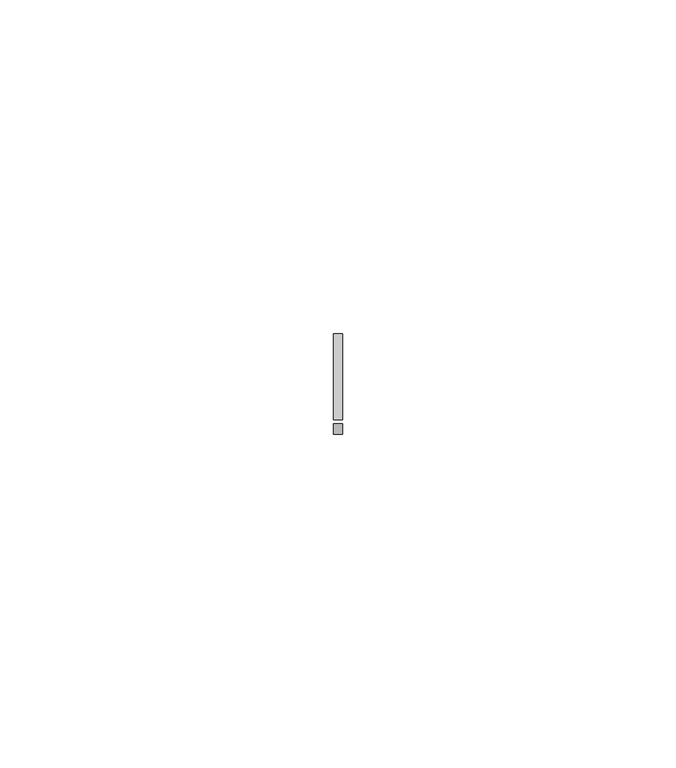
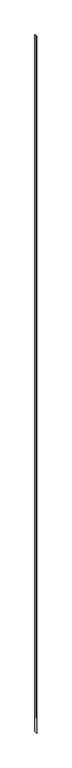
"""IFC4 building model written with IfcOpenShell, lengths in millimetres: proxy geometry, Generic Models 11:Generic Models 1:306267:Generic Models 1:306267 : Generic Models 11:Generic Models 1:306267:300405:Generic Models 1:306267:Generic Models 1:306267 : Generic Models 11:Generic Models 1:306267:300405 : Generic Models 11:Generic Models 1:306267:Generic Models 1:306267 : Generic Models 11:Generic Models 1:306267:300405:31 : Generic Models 11:Generic Models 1:306267:Generic Models 1:306267 : Generic Models 11:Generic Models 1:306267:300405:Generic Models 1:306267:Generic Models 1:306267 : Generic Models 11:Generic Models 1:306267:300405 : Generic Models 11:Generic Models 1:306267:Generic Models 1:306267 : Generic Models 11:Generic Models 1:306267:300405:300182."""

from ifc_helpers import new_model, si_unit, frame, origin, place, context, project, spatial, polyline, outline, extrude, source, transform, mapped, element, save


def generic_models_74956f50(model_context):
    return source(origin(), model_context, "Body", "SweptSolid", [
        extrude(outline(polyline([(-579016.1920851, 0.0), (-579030.680779, 0.0), (-579030.680779, 78.871332), (-579029.093279, 81.1385169), (-579029.093279, 3689.35), (-579016.1920851, 3689.35), (-579016.1920851, 0.0)])), frame((596182.8367239, 0.0, 0.0), z_axis=(1.0, 0.0, 0.0), x_axis=(0.0, 1.0, 0.0)), (0.0, 0.0, 1.0), 1.3607676),
    ])


if __name__ == "__main__":
    model = new_model("IFC4")
    model_context = context("Model", 3, world=origin())
    ifc_project = project(units=[si_unit("LENGTHUNIT", "METRE", prefix="MILLI")], contexts=[model_context])
    site = spatial("IfcSite", under=ifc_project)
    building = spatial("IfcBuilding", under=site)
    placement = place(None, origin())
    generic_models_shape = generic_models_74956f50(model_context)
    element("IfcBuildingElementProxy", 1, Name="Generic Models 11:Generic Models 1:306267:Generic Models 1:306267 : Generic Models 11:Generic Models 1:306267:300405:Generic Models 1:306267:Generic Models 1:306267 : Generic Models 11:Generic Models 1:306267:300405 : Generic Models 11:Generic Models 1:306267:Generic Models 1:306267 : Generic Models 11:Generic Models 1:306267:300405:31 : Generic Models 11:Generic Models 1:306267:Generic Models 1:306267 : Generic Models 11:Generic Models 1:306267:300405:Generic Models 1:306267:Generic Models 1:306267 : Generic Models 11:Generic Models 1:306267:300405 : Generic Models 11:Generic Models 1:306267:Generic Models 1:306267 : Generic Models 11:Generic Models 1:306267:300405:300182", ObjectType="Generic Models 11:Generic Models 1:306267:Generic Models 1:306267 : Generic Models 11:Generic Models 1:306267:300405:Generic Models 1:306267:Generic Models 1:306267 : Generic Models 11:Generic Models 1:306267:300405 : Generic Models 11:Generic Models 1:306267:Generic Models 1:306267 : Generic Models 11:Generic Models 1:306267:300405:31 : Generic Models 11:Generic Models 1:306267:Generic Models 1:306267 : Generic Models 11:Generic Models 1:306267:300405:Generic Models 1:306267:Generic Models 1:306267 : Generic Models 11:Generic Models 1:306267:300405 : Generic Models 11:Generic Models 1:306267:Generic Models 1:306267 : Generic Models 11:Generic Models 1:306267:300405:300182", at=placement, inside=building, context=model_context, shape_type="MappedRepresentation", body=[
        mapped(generic_models_shape, transform((0.0, 0.0, 0.0), x_axis=(1.0, 0.0, 0.0), y_axis=(0.0, 1.0, 0.0), z_axis=(0.0, 0.0, 1.0))),
    ])
    save(model, "model.ifc")

# Revit data of these elements
# Type "Generic Models 11:Generic Models 1:306267:Generic Models 1:306267 : Generic Models 11:Generic Models 1:306267:300405:Generic Models 1:306267:Generic Models 1:306267 : Generic Models 11:Generic Models 1:306267:300405 : Generic Models 11:Generic Models 1:306267:Generic Models 1:306267 : Generic Models 11:Generic Models 1:306267:300405:31 : Generic Models 11:Generic Models 1:306267:Generic Models 1:306267 : Generic Models 11:Generic Models 1:306267:300405:Generic Models 1:306267:Generic Models 1:306267 : Generic Models 11:Generic Models 1:306267:300405 : Generic Models 11:Generic Models 1:306267:Generic Models 1:306267 : Generic Models 11:Generic Models 1:306267:300405:300182"
#   NameOverride = "Generic Models 11:Generic Models 1:306267:Generic Models 1:306267 : Generic Models 11:Generic Models 1:306267:300405:Generic Models 1:306267:Generic Models 1:306267 : Generic Models 11:Generic Models 1:306267:300405 : Generic Models 11:Generic Models 1:306267:Generic Models 1:306267 : Generic Models 11:Generic Models 1:306267:300405:300182"
#   ObjectTypeOverride = "Generic Models 1:306267:Generic Models 1:306267 : Generic Models 11:Generic Models 1:306267:300405 : Generic Models 11:Generic Models 1:306267:Generic Models 1:306267 : Generic Models 11:Generic Models 1:306267:300405"
#   Reference = "Generic Models 1"
#   Tag = "300182"
# Element 1 (IfcBuildingElementProxy, "Generic Models 11:Generic Models 1:306267:Generic Models 1:306267 : Generic Models 11:Generic Models 1:306267:300405:Generic Models 1:306267:Generic Models 1:306267 : Generic Models 11:Generic Models 1:306267:300405 : Generic Models 11:Generic Models 1:306267:Generic Models 1:306267 : Generic Models 11:Generic Models 1:306267:300405:31 : Generic Models 11:Generic Models 1:306267:Generic Models 1:306267 : Generic Models 11:Generic Models 1:306267:300405:Generic Models 1:306267:Generic Models 1:306267 : Generic Models 11:Generic Models 1:306267:300405 : Generic Models 11:Generic Models 1:306267:Generic Models 1:306267 : Generic Models 11:Generic Models 1:306267:300405:300182")
#   Materials on its faces: "UV STABLE WATER RESISTANT VAPOR PERMEABLE AIR BARRIER (WRB) - WRAP JAMBS/HEADERS - BLACK COLOR"
# Materials
#   "UV STABLE WATER RESISTANT VAPOR PERMEABLE AIR BARRIER (WRB) - WRAP JAMBS/HEADERS - BLACK COLOR": class "Generic", colour RGB 51 162 45, transparency 0, Description = "Polyethylene film membrane", Cost = 0
